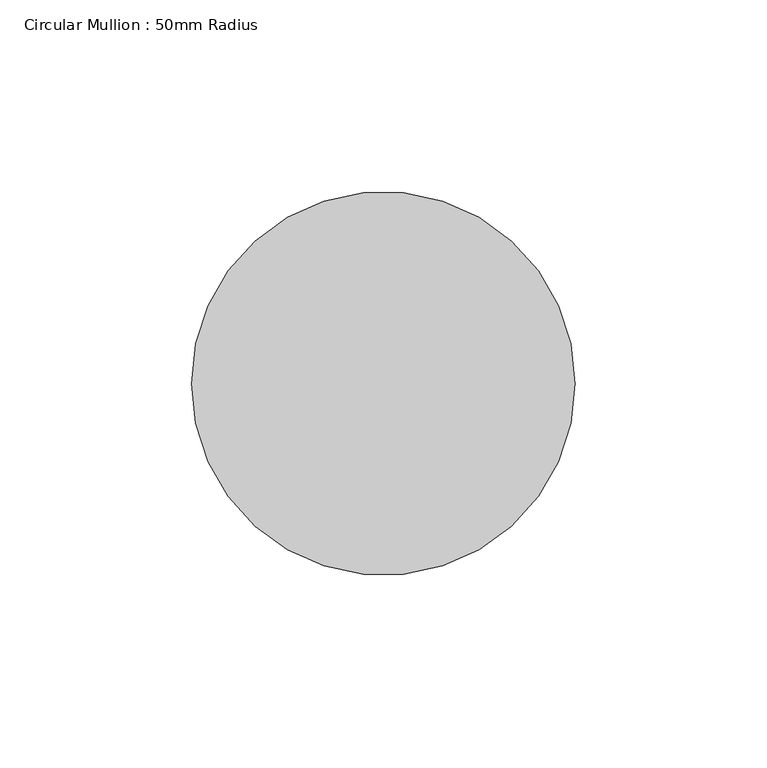
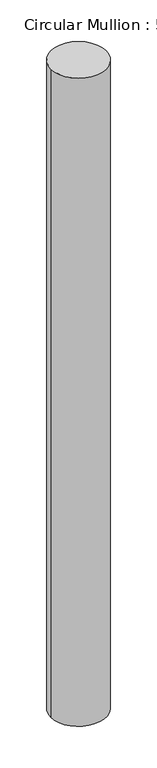
"""IFC4 building model written with IfcOpenShell, lengths in millimetres: member geometry, Circular Mullion : 50mm Radius."""

from ifc_helpers import new_model, si_unit, point, frame, origin, origin_2d, place, context, project, spatial, circle_curve, trimmed, segment, composite_curve, outline, extrude, source, transform, mapped, element, save


def circular_mullion_50mm_radius_1439f9c9(model_context):
    return source(origin(), model_context, "Body", "SweptSolid", [
        extrude(outline(composite_curve([segment(trimmed(circle_curve(origin_2d(), 50.0), [point((50.0, 0.0))], [point((-50.0, 0.0))], False, "CARTESIAN"), True, "CONTINUOUS"), segment(trimmed(circle_curve(origin_2d(), 50.0), [point((-50.0, 0.0))], [point((50.0, 0.0))], False, "CARTESIAN"), True, "CONTINUOUS")], self_intersect=False)), frame((0.0, 0.0, -1241.5463488), z_axis=(0.0, 0.0, 1.0), x_axis=(1.0, 0.0, 0.0)), (0.0, 0.0, 1.0), 1241.5463488),
    ])


if __name__ == "__main__":
    model = new_model("IFC4")
    model_context = context("Model", 3, world=origin())
    ifc_project = project(units=[si_unit("LENGTHUNIT", "METRE", prefix="MILLI")], contexts=[model_context])
    site = spatial("IfcSite", under=ifc_project)
    building = spatial("IfcBuilding", under=site)
    placement = place(None, origin())
    circular_mullion_50mm_radius_shape = circular_mullion_50mm_radius_1439f9c9(model_context)
    element("IfcMember", 1, ObjectType="Circular Mullion : 50mm Radius", at=placement, inside=building, context=model_context, shape_type="MappedRepresentation", body=[
        mapped(circular_mullion_50mm_radius_shape, transform((0.0, 0.0, 0.0), x_axis=(1.0, 0.0, 0.0), y_axis=(0.0, 1.0, 0.0), z_axis=(0.0, 0.0, 1.0))),
    ])
    save(model, "model.ifc")

# Revit data of these elements
# Type "Circular Mullion : 50mm Radius"
#   built-in parameter 1007350 = 0.164042 (stored number, unit not read)
# Element 1 (IfcMember, "Circular Mullion : 50mm Radius")
#   Materials on its faces: "Aluminium"
# Materials
#   "Aluminium": class "Metal", colour RGB 247 247 247, transparency 0, Description = "Aluminium 6061", Cost = 0
